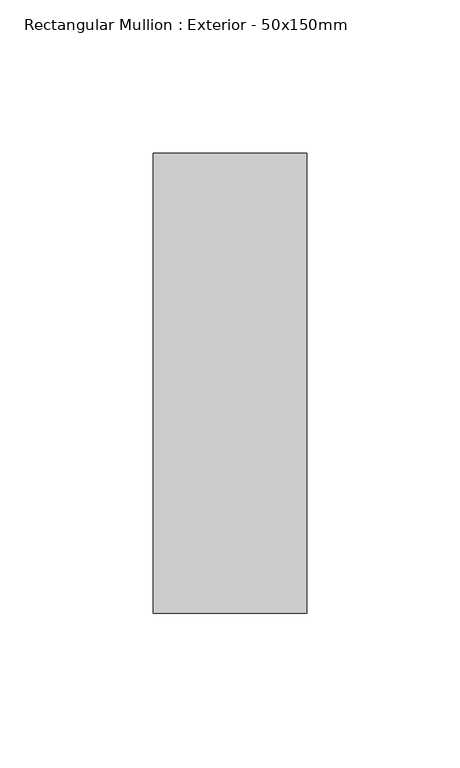
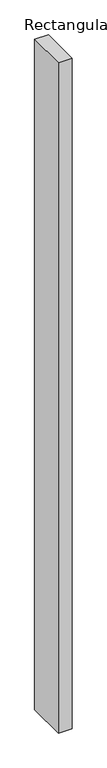
"""IFC4 building model written with IfcOpenShell, lengths in millimetres: member geometry, Rectangular Mullion : Exterior - 50x150mm."""

from ifc_helpers import new_model, si_unit, frame, origin, place, context, project, spatial, polyline, outline, extrude, source, transform, mapped, element, save


def rectangular_mullion_exterior_50x150mm_9e283e44(model_context):
    return source(origin(), model_context, "Body", "SweptSolid", [
        extrude(outline(polyline([(0.0, 0.0), (0.0, -150.0), (-50.0, -150.0), (-50.0, 0.0), (0.0, 0.0)])), frame((0.0, 0.0, -2600.0), z_axis=(0.0, 0.0, 1.0), x_axis=(1.0, 0.0, 0.0)), (0.0, 0.0, 1.0), 2600.0),
    ])


if __name__ == "__main__":
    model = new_model("IFC4")
    model_context = context("Model", 3, world=origin())
    ifc_project = project(units=[si_unit("LENGTHUNIT", "METRE", prefix="MILLI")], contexts=[model_context])
    site = spatial("IfcSite", under=ifc_project)
    building = spatial("IfcBuilding", under=site)
    placement = place(None, origin())
    rectangular_mullion_exterior_50x150mm_shape = rectangular_mullion_exterior_50x150mm_9e283e44(model_context)
    element("IfcMember", 1, ObjectType="Rectangular Mullion : Exterior - 50x150mm", at=placement, inside=building, context=model_context, shape_type="MappedRepresentation", body=[
        mapped(rectangular_mullion_exterior_50x150mm_shape, transform((0.0, 0.0, 0.0), x_axis=(1.0, 0.0, 0.0), y_axis=(0.0, 1.0, 0.0), z_axis=(0.0, 0.0, 1.0))),
    ])
    save(model, "model.ifc")

# Revit data of these elements
# Type "Rectangular Mullion : Exterior - 50x150mm"
#   built-in parameter 1007351 = -0.246063 (stored number, unit not read)
#   built-in parameter 1007304 = 0.492126 (stored number, unit not read)
#   built-in parameter 1007301 = 0.082021 (stored number, unit not read)
#   built-in parameter 1007300 = 0.082021 (stored number, unit not read)
# Element 1 (IfcMember, "Rectangular Mullion : Exterior - 50x150mm")
#   Materials on its faces: "Default Frame/Mullion (Interior/Exterior)"
# Materials
#   "Default Frame/Mullion (Interior/Exterior)": class "Generic", colour RGB 205 205 205, transparency 0, Description = "Udefineret karm/ramme materiale", Cost = 0
